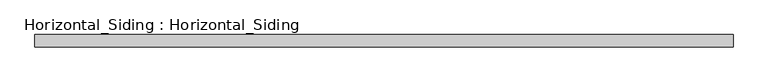
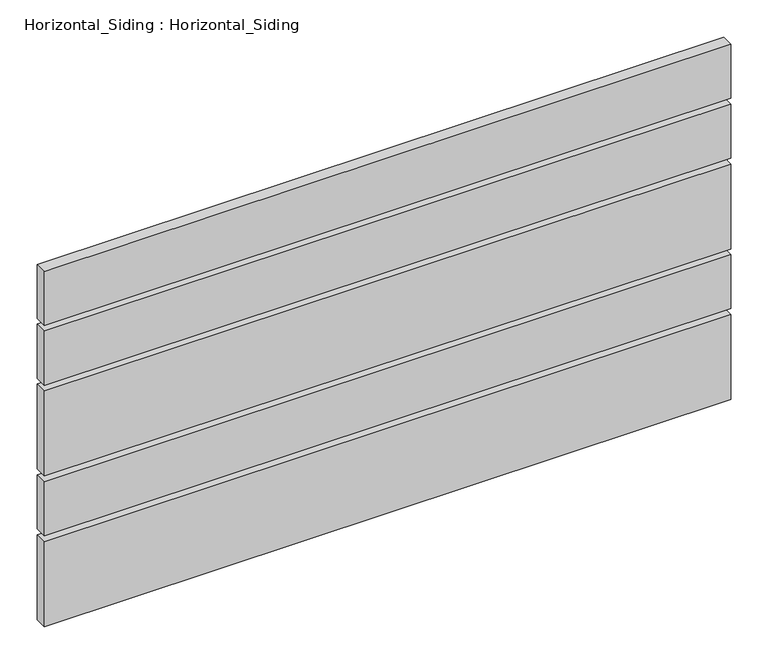
"""IFC4 building model written with IfcOpenShell, lengths in millimetres: plate geometry, Horizontal_Siding : Horizontal_Siding."""

import ifcopenshell
import ifcopenshell.guid

model = None  # the IFC model being written
_history = None  # IfcOwnerHistory: only IFC2X3 demands one
_inside = {}  # id of a spatial element -> (the spatial element, [elements in it])
_under = {}  # id of a project, library or spatial element -> (it, [spatial elements below it])
_declared = {}  # id of a project -> (the project, [libraries it declares])
_typed = {}  # id of a type object -> (the type object, [elements of that type])
_made_of = {}  # id of a material, layer set ... -> (it, [elements and type objects made of it])


def new_model(schema):
    """Start an empty IFC model of exactly this schema.

    Asked for "IFC4X3", IfcOpenShell would pick the latest addendum, in which some entities
    have other attributes; the version numbers below select the first issue.
    IFC2X3 requires an IfcOwnerHistory on every rooted entity: one is made here for all.
    """
    global model, _history
    if schema == "IFC4X3":
        model = ifcopenshell.file(schema_version=(4, 3, 0, 0))
    else:
        model = ifcopenshell.file(schema=schema)
    _inside.clear()
    _under.clear()
    _declared.clear()
    _typed.clear()
    _made_of.clear()
    _history = None
    if model.schema == "IFC2X3":
        org = make("IfcOrganization", Name="unknown")
        user = make(
            "IfcPersonAndOrganization",
            ThePerson=make("IfcPerson", FamilyName="unknown"),
            TheOrganization=org,
        )
        app = make(
            "IfcApplication",
            ApplicationDeveloper=org,
            Version="unknown",
            ApplicationFullName="unknown",
            ApplicationIdentifier="unknown",
        )
        _history = make(
            "IfcOwnerHistory",
            OwningUser=user,
            OwningApplication=app,
            ChangeAction="ADDED",
            CreationDate=0,
        )
    return model


def make(cls, **values):
    """One entity of the class cls with the attributes given. An attribute that is None is left unset."""
    return model.create_entity(
        cls, **{name: value for name, value in values.items() if value is not None}
    )


def rooted(cls, **values):
    """An entity with a GlobalId (a new one), such as an element, a storey or a relation."""
    return make(cls, GlobalId=ifcopenshell.guid.new(), OwnerHistory=_history, **values)


def si_unit(unit_type, name, prefix=None):
    """IfcSIUnit, for example si_unit("LENGTHUNIT", "METRE", prefix="MILLI")."""
    return make("IfcSIUnit", UnitType=unit_type, Prefix=prefix, Name=name)


def assignment(units):
    """IfcUnitAssignment: the units of a project."""
    return None if units is None else make("IfcUnitAssignment", Units=units)


def point(xyz):
    """IfcCartesianPoint."""
    return None if xyz is None else make("IfcCartesianPoint", Coordinates=xyz)


def direction(xyz):
    """IfcDirection."""
    return None if xyz is None else make("IfcDirection", DirectionRatios=xyz)


def frame(location, z_axis=None, x_axis=None):
    """IfcAxis2Placement3D, a coordinate frame: its origin and axes. An axis left out is left unset."""
    return make(
        "IfcAxis2Placement3D",
        Location=point(location),
        Axis=direction(z_axis),
        RefDirection=direction(x_axis),
    )


def origin():
    """The frame at (0, 0, 0) with its axes left unset."""
    return frame((0.0, 0.0, 0.0))


def place(relative_to, where):
    """IfcLocalPlacement: puts the frame where relative to a parent placement (None: the world)."""
    return make(
        "IfcLocalPlacement", PlacementRelTo=relative_to, RelativePlacement=where
    )


def context(
    kind, dimensions, precision=None, world=None, true_north=None, identifier=None
):
    """IfcGeometricRepresentationContext, for example the 3D "Model" context."""
    return make(
        "IfcGeometricRepresentationContext",
        ContextIdentifier=identifier,
        ContextType=kind,
        CoordinateSpaceDimension=dimensions,
        Precision=precision,
        WorldCoordinateSystem=world,
        TrueNorth=true_north,
    )


def project(units=None, contexts=None):
    """IfcProject with its units and contexts."""
    return rooted(
        "IfcProject",
        Name="project",
        RepresentationContexts=contexts,
        UnitsInContext=assignment(units),
    )


def spatial(cls, under=None, at=None, **own):
    """A site, building, storey or space (cls), placed at a placement, below another one or the project."""
    s = rooted(cls, ObjectPlacement=at, **own)
    if under is not None:
        _under.setdefault(under.id(), (under, []))[1].append(s)
    return s


def polyline(points):
    """IfcPolyline through the points."""
    return make("IfcPolyline", Points=[point(p) for p in points])


def outline(outer, holes=None, kind="AREA"):
    """IfcArbitraryClosedProfileDef: a profile drawn as a closed curve; with holes, ...WithVoids."""
    if holes is None:
        return make("IfcArbitraryClosedProfileDef", ProfileType=kind, OuterCurve=outer)
    return make(
        "IfcArbitraryProfileDefWithVoids",
        ProfileType=kind,
        OuterCurve=outer,
        InnerCurves=holes,
    )


def extrude(swept, where, along, depth):
    """IfcExtrudedAreaSolid: the profile swept, set in the frame where, extruded along a direction by depth."""
    return make(
        "IfcExtrudedAreaSolid",
        SweptArea=swept,
        Position=where,
        ExtrudedDirection=direction(along),
        Depth=depth,
    )


def shape(context_of_items, identifier, shape_type, items):
    """IfcShapeRepresentation: the items that make up one representation, for example the "Body"."""
    return make(
        "IfcShapeRepresentation",
        ContextOfItems=context_of_items,
        RepresentationIdentifier=identifier,
        RepresentationType=shape_type,
        Items=items,
    )


def source(mapping_origin, context_of_items, identifier, shape_type, items):
    """IfcRepresentationMap: a shape defined once, which mapped items show again and again."""
    return make(
        "IfcRepresentationMap",
        MappingOrigin=mapping_origin,
        MappedRepresentation=shape(context_of_items, identifier, shape_type, items),
    )


def transform(
    local_origin,
    x_axis=None,
    y_axis=None,
    z_axis=None,
    scale=None,
    scale2=None,
    scale3=None,
    uniform=True,
):
    """IfcCartesianTransformationOperator3D, or its non-uniform kind. x_axis, y_axis, z_axis: its Axis1, 2, 3."""
    if uniform:
        return make(
            "IfcCartesianTransformationOperator3D",
            Axis1=direction(x_axis),
            Axis2=direction(y_axis),
            LocalOrigin=point(local_origin),
            Scale=scale,
            Axis3=direction(z_axis),
        )
    return make(
        "IfcCartesianTransformationOperator3DnonUniform",
        Axis1=direction(x_axis),
        Axis2=direction(y_axis),
        LocalOrigin=point(local_origin),
        Scale=scale,
        Axis3=direction(z_axis),
        Scale2=scale2,
        Scale3=scale3,
    )


def mapped(mapping_source, mapping_target):
    """IfcMappedItem: shows the shape of a source again, moved by a transform."""
    return make(
        "IfcMappedItem", MappingSource=mapping_source, MappingTarget=mapping_target
    )


def made_of(thing, what):
    """Note that an element or type object is made of a material, layer set ...; save() writes the relation."""
    if what is not None:
        _made_of.setdefault(what.id(), (what, []))[1].append(thing)
    return thing


def element(
    cls,
    number,
    at=None,
    inside=None,
    cuts=None,
    type_object=None,
    material=None,
    context=None,
    identifier="Body",
    shape_type=None,
    held_by="IfcProductDefinitionShape",
    body=None,
    shapes=None,
    **own,
):
    """One element of the class cls, such as IfcWall. Its Tag is "e" and its number.

    at: its placement. inside: the storey or other place that contains it. cuts: it is an
    opening in that element (IfcRelVoidsElement). A single representation is given by context,
    identifier, shape_type and body (its items); several are given by shapes. held_by: the class
    of the entity that holds the representations. save() writes the other relations.
    """
    e = rooted(cls, Tag="e%d" % number, ObjectPlacement=at, **own)
    if body is not None:
        shapes = [shape(context, identifier, shape_type, body)]
    if shapes is not None:
        e.Representation = make(held_by, Representations=shapes)
    if inside is not None:
        _inside.setdefault(inside.id(), (inside, []))[1].append(e)
    if cuts is not None:
        rooted(
            "IfcRelVoidsElement", RelatingBuildingElement=cuts, RelatedOpeningElement=e
        )
    if type_object is not None:
        _typed.setdefault(type_object.id(), (type_object, []))[1].append(e)
    return made_of(e, material)


def aggregate(whole, parts):
    """IfcRelAggregates: a whole, such as a stair, and the parts it consists of."""
    return rooted("IfcRelAggregates", RelatingObject=whole, RelatedObjects=parts)


def save(model, path):
    """Write the relations noted so far, then the file.

    IfcRelAggregates (storeys below a building ...), IfcRelContainedInSpatialStructure (elements
    in a storey), IfcRelDefinesByType, IfcRelAssociatesMaterial and IfcRelDeclares: one each for
    every whole, place, type object, material and project.
    """
    for whole, parts in _under.values():
        aggregate(whole, parts)
    for where, things in _inside.values():
        rooted(
            "IfcRelContainedInSpatialStructure",
            RelatedElements=things,
            RelatingStructure=where,
        )
    for kind, things in _typed.values():
        rooted("IfcRelDefinesByType", RelatedObjects=things, RelatingType=kind)
    for what, things in _made_of.values():
        rooted("IfcRelAssociatesMaterial", RelatedObjects=things, RelatingMaterial=what)
    for by, libraries in _declared.values():
        rooted("IfcRelDeclares", RelatingContext=by, RelatedDefinitions=libraries)
    model.write(path)


def horizontal_siding_horizontal_siding_6226d231(model_context):
    return source(origin(), model_context, "Body", "SweptSolid", [
        extrude(outline(polyline([(533.4, -19.05), (-533.4, -19.05), (-533.4, 0.0), (533.4, 0.0), (533.4, -19.05)])), frame((0.0, 0.0, 9.525), z_axis=(0.0, 0.0, 1.0), x_axis=(1.0, 0.0, 0.0)), (0.0, 0.0, 1.0), 139.7),
        extrude(outline(polyline([(533.4, -19.05), (-533.4, -19.05), (-533.4, 0.0), (533.4, 0.0), (533.4, -19.05)])), frame((0.0, 0.0, 158.75), z_axis=(0.0, 0.0, 1.0), x_axis=(1.0, 0.0, 0.0)), (0.0, 0.0, 1.0), 88.9),
        extrude(outline(polyline([(533.4, -19.05), (-533.4, -19.05), (-533.4, 0.0), (533.4, 0.0), (533.4, -19.05)])), frame((0.0, 0.0, 257.175), z_axis=(0.0, 0.0, 1.0), x_axis=(1.0, 0.0, 0.0)), (0.0, 0.0, 1.0), 139.7),
        extrude(outline(polyline([(533.4, -19.05), (-533.4, -19.05), (-533.4, 0.0), (533.4, 0.0), (533.4, -19.05)])), frame((0.0, 0.0, 406.4), z_axis=(0.0, 0.0, 1.0), x_axis=(1.0, 0.0, 0.0)), (0.0, 0.0, 1.0), 88.9),
        extrude(outline(polyline([(533.4, -19.05), (-533.4, -19.05), (-533.4, 0.0), (533.4, 0.0), (533.4, -19.05)])), frame((0.0, 0.0, 504.825), z_axis=(0.0, 0.0, 1.0), x_axis=(1.0, 0.0, 0.0)), (0.0, 0.0, 1.0), 88.9),
    ])


if __name__ == "__main__":
    model = new_model("IFC4")
    model_context = context("Model", 3, world=origin())
    ifc_project = project(units=[si_unit("LENGTHUNIT", "METRE", prefix="MILLI")], contexts=[model_context])
    site = spatial("IfcSite", under=ifc_project)
    building = spatial("IfcBuilding", under=site)
    placement = place(None, origin())
    horizontal_siding_horizontal_siding_shape = horizontal_siding_horizontal_siding_6226d231(model_context)
    element("IfcPlate", 1, ObjectType="Horizontal_Siding : Horizontal_Siding", at=placement, inside=building, context=model_context, shape_type="MappedRepresentation", body=[
        mapped(horizontal_siding_horizontal_siding_shape, transform((0.0, 0.0, 0.0), x_axis=(1.0, 0.0, 0.0), y_axis=(0.0, 1.0, 0.0), z_axis=(0.0, 0.0, 1.0))),
    ])
    save(model, "model.ifc")

# Revit data of these elements
# Type "Horizontal_Siding : Horizontal_Siding"
#   Analytic Construction = "<None>"
#   extend = 0' - 2 3/4"
#   Width_2 = 0' - 3 1/2"
#   Width_1 = 0' - 5 1/2"
#   Gap = 0' - 0 3/8"
#   Plank Material = SLOTTED WOOD FENCE (THERMALLY MODIFIED WOOD: ARBOR WOOD)\n(EXTERIOR STAIN : PENOFIN VERDE EXT. STAIN - COLOR: CEDAR)
# Element 1 (IfcPlate, "Horizontal_Siding : Horizontal_Siding")
#   Materials on its faces: "SLOTTED WOOD FENCE (THERMALLY MODIFIED WOOD: ARBOR WOOD)\n(EXTERIOR STAIN : PENOFIN VERDE EXT. STAIN - COLOR: CEDAR)"
# Materials
#   "SLOTTED WOOD FENCE (THERMALLY MODIFIED WOOD: ARBOR WOOD)\n(EXTERIOR STAIN : PENOFIN VERDE EXT. STAIN - COLOR: CEDAR)": class "Wood", colour RGB 164 134 123, transparency 0, Description = "Pinus Echinata", Cost = 0
